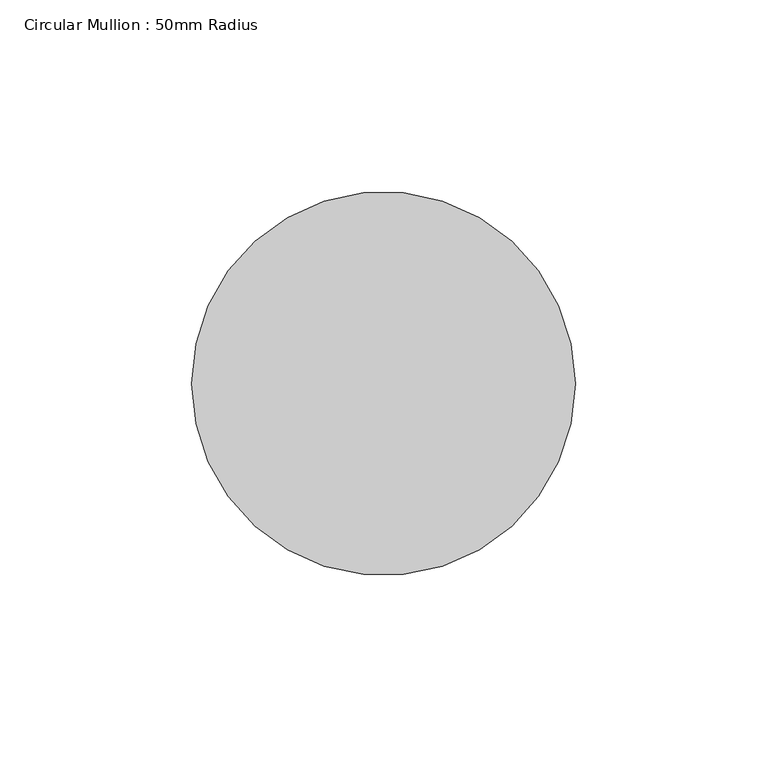
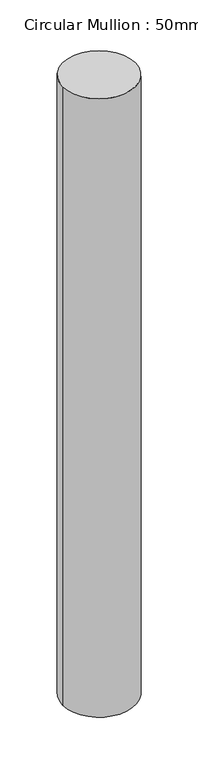
"""IFC4 building model written with IfcOpenShell, lengths in millimetres: member geometry, Circular Mullion : 50mm Radius."""

import ifcopenshell
import ifcopenshell.guid

model = None  # the IFC model being written
_history = None  # IfcOwnerHistory: only IFC2X3 demands one
_inside = {}  # id of a spatial element -> (the spatial element, [elements in it])
_under = {}  # id of a project, library or spatial element -> (it, [spatial elements below it])
_declared = {}  # id of a project -> (the project, [libraries it declares])
_typed = {}  # id of a type object -> (the type object, [elements of that type])
_made_of = {}  # id of a material, layer set ... -> (it, [elements and type objects made of it])


def new_model(schema):
    """Start an empty IFC model of exactly this schema.

    Asked for "IFC4X3", IfcOpenShell would pick the latest addendum, in which some entities
    have other attributes; the version numbers below select the first issue.
    IFC2X3 requires an IfcOwnerHistory on every rooted entity: one is made here for all.
    """
    global model, _history
    if schema == "IFC4X3":
        model = ifcopenshell.file(schema_version=(4, 3, 0, 0))
    else:
        model = ifcopenshell.file(schema=schema)
    _inside.clear()
    _under.clear()
    _declared.clear()
    _typed.clear()
    _made_of.clear()
    _history = None
    if model.schema == "IFC2X3":
        org = make("IfcOrganization", Name="unknown")
        user = make(
            "IfcPersonAndOrganization",
            ThePerson=make("IfcPerson", FamilyName="unknown"),
            TheOrganization=org,
        )
        app = make(
            "IfcApplication",
            ApplicationDeveloper=org,
            Version="unknown",
            ApplicationFullName="unknown",
            ApplicationIdentifier="unknown",
        )
        _history = make(
            "IfcOwnerHistory",
            OwningUser=user,
            OwningApplication=app,
            ChangeAction="ADDED",
            CreationDate=0,
        )
    return model


def make(cls, **values):
    """One entity of the class cls with the attributes given. An attribute that is None is left unset."""
    return model.create_entity(
        cls, **{name: value for name, value in values.items() if value is not None}
    )


def rooted(cls, **values):
    """An entity with a GlobalId (a new one), such as an element, a storey or a relation."""
    return make(cls, GlobalId=ifcopenshell.guid.new(), OwnerHistory=_history, **values)


def si_unit(unit_type, name, prefix=None):
    """IfcSIUnit, for example si_unit("LENGTHUNIT", "METRE", prefix="MILLI")."""
    return make("IfcSIUnit", UnitType=unit_type, Prefix=prefix, Name=name)


def assignment(units):
    """IfcUnitAssignment: the units of a project."""
    return None if units is None else make("IfcUnitAssignment", Units=units)


def point(xyz):
    """IfcCartesianPoint."""
    return None if xyz is None else make("IfcCartesianPoint", Coordinates=xyz)


def direction(xyz):
    """IfcDirection."""
    return None if xyz is None else make("IfcDirection", DirectionRatios=xyz)


def frame(location, z_axis=None, x_axis=None):
    """IfcAxis2Placement3D, a coordinate frame: its origin and axes. An axis left out is left unset."""
    return make(
        "IfcAxis2Placement3D",
        Location=point(location),
        Axis=direction(z_axis),
        RefDirection=direction(x_axis),
    )


def frame_2d(location, x_axis=None):
    """IfcAxis2Placement2D, a coordinate frame in the plane: its origin and x axis."""
    return make(
        "IfcAxis2Placement2D", Location=point(location), RefDirection=direction(x_axis)
    )


def origin():
    """The frame at (0, 0, 0) with its axes left unset."""
    return frame((0.0, 0.0, 0.0))


def origin_2d():
    """The frame at (0, 0) in the plane with its x axis left unset."""
    return frame_2d((0.0, 0.0))


def place(relative_to, where):
    """IfcLocalPlacement: puts the frame where relative to a parent placement (None: the world)."""
    return make(
        "IfcLocalPlacement", PlacementRelTo=relative_to, RelativePlacement=where
    )


def context(
    kind, dimensions, precision=None, world=None, true_north=None, identifier=None
):
    """IfcGeometricRepresentationContext, for example the 3D "Model" context."""
    return make(
        "IfcGeometricRepresentationContext",
        ContextIdentifier=identifier,
        ContextType=kind,
        CoordinateSpaceDimension=dimensions,
        Precision=precision,
        WorldCoordinateSystem=world,
        TrueNorth=true_north,
    )


def project(units=None, contexts=None):
    """IfcProject with its units and contexts."""
    return rooted(
        "IfcProject",
        Name="project",
        RepresentationContexts=contexts,
        UnitsInContext=assignment(units),
    )


def spatial(cls, under=None, at=None, **own):
    """A site, building, storey or space (cls), placed at a placement, below another one or the project."""
    s = rooted(cls, ObjectPlacement=at, **own)
    if under is not None:
        _under.setdefault(under.id(), (under, []))[1].append(s)
    return s


def circle_curve(where, radius):
    """IfcCircle in the frame where."""
    return make("IfcCircle", Position=where, Radius=radius)


def trimmed(basis, trim1, trim2, sense, master):
    """IfcTrimmedCurve: the piece of a basis curve between two trims."""
    return make(
        "IfcTrimmedCurve",
        BasisCurve=basis,
        Trim1=trim1,
        Trim2=trim2,
        SenseAgreement=sense,
        MasterRepresentation=master,
    )


def segment(curve, same_sense, transition):
    """IfcCompositeCurveSegment."""
    return make(
        "IfcCompositeCurveSegment",
        Transition=transition,
        SameSense=same_sense,
        ParentCurve=curve,
    )


def composite_curve(segments, self_intersect=None):
    """IfcCompositeCurve: segments joined end to end."""
    return make("IfcCompositeCurve", Segments=segments, SelfIntersect=self_intersect)


def outline(outer, holes=None, kind="AREA"):
    """IfcArbitraryClosedProfileDef: a profile drawn as a closed curve; with holes, ...WithVoids."""
    if holes is None:
        return make("IfcArbitraryClosedProfileDef", ProfileType=kind, OuterCurve=outer)
    return make(
        "IfcArbitraryProfileDefWithVoids",
        ProfileType=kind,
        OuterCurve=outer,
        InnerCurves=holes,
    )


def extrude(swept, where, along, depth):
    """IfcExtrudedAreaSolid: the profile swept, set in the frame where, extruded along a direction by depth."""
    return make(
        "IfcExtrudedAreaSolid",
        SweptArea=swept,
        Position=where,
        ExtrudedDirection=direction(along),
        Depth=depth,
    )


def shape(context_of_items, identifier, shape_type, items):
    """IfcShapeRepresentation: the items that make up one representation, for example the "Body"."""
    return make(
        "IfcShapeRepresentation",
        ContextOfItems=context_of_items,
        RepresentationIdentifier=identifier,
        RepresentationType=shape_type,
        Items=items,
    )


def source(mapping_origin, context_of_items, identifier, shape_type, items):
    """IfcRepresentationMap: a shape defined once, which mapped items show again and again."""
    return make(
        "IfcRepresentationMap",
        MappingOrigin=mapping_origin,
        MappedRepresentation=shape(context_of_items, identifier, shape_type, items),
    )


def transform(
    local_origin,
    x_axis=None,
    y_axis=None,
    z_axis=None,
    scale=None,
    scale2=None,
    scale3=None,
    uniform=True,
):
    """IfcCartesianTransformationOperator3D, or its non-uniform kind. x_axis, y_axis, z_axis: its Axis1, 2, 3."""
    if uniform:
        return make(
            "IfcCartesianTransformationOperator3D",
            Axis1=direction(x_axis),
            Axis2=direction(y_axis),
            LocalOrigin=point(local_origin),
            Scale=scale,
            Axis3=direction(z_axis),
        )
    return make(
        "IfcCartesianTransformationOperator3DnonUniform",
        Axis1=direction(x_axis),
        Axis2=direction(y_axis),
        LocalOrigin=point(local_origin),
        Scale=scale,
        Axis3=direction(z_axis),
        Scale2=scale2,
        Scale3=scale3,
    )


def mapped(mapping_source, mapping_target):
    """IfcMappedItem: shows the shape of a source again, moved by a transform."""
    return make(
        "IfcMappedItem", MappingSource=mapping_source, MappingTarget=mapping_target
    )


def made_of(thing, what):
    """Note that an element or type object is made of a material, layer set ...; save() writes the relation."""
    if what is not None:
        _made_of.setdefault(what.id(), (what, []))[1].append(thing)
    return thing


def element(
    cls,
    number,
    at=None,
    inside=None,
    cuts=None,
    type_object=None,
    material=None,
    context=None,
    identifier="Body",
    shape_type=None,
    held_by="IfcProductDefinitionShape",
    body=None,
    shapes=None,
    **own,
):
    """One element of the class cls, such as IfcWall. Its Tag is "e" and its number.

    at: its placement. inside: the storey or other place that contains it. cuts: it is an
    opening in that element (IfcRelVoidsElement). A single representation is given by context,
    identifier, shape_type and body (its items); several are given by shapes. held_by: the class
    of the entity that holds the representations. save() writes the other relations.
    """
    e = rooted(cls, Tag="e%d" % number, ObjectPlacement=at, **own)
    if body is not None:
        shapes = [shape(context, identifier, shape_type, body)]
    if shapes is not None:
        e.Representation = make(held_by, Representations=shapes)
    if inside is not None:
        _inside.setdefault(inside.id(), (inside, []))[1].append(e)
    if cuts is not None:
        rooted(
            "IfcRelVoidsElement", RelatingBuildingElement=cuts, RelatedOpeningElement=e
        )
    if type_object is not None:
        _typed.setdefault(type_object.id(), (type_object, []))[1].append(e)
    return made_of(e, material)


def aggregate(whole, parts):
    """IfcRelAggregates: a whole, such as a stair, and the parts it consists of."""
    return rooted("IfcRelAggregates", RelatingObject=whole, RelatedObjects=parts)


def save(model, path):
    """Write the relations noted so far, then the file.

    IfcRelAggregates (storeys below a building ...), IfcRelContainedInSpatialStructure (elements
    in a storey), IfcRelDefinesByType, IfcRelAssociatesMaterial and IfcRelDeclares: one each for
    every whole, place, type object, material and project.
    """
    for whole, parts in _under.values():
        aggregate(whole, parts)
    for where, things in _inside.values():
        rooted(
            "IfcRelContainedInSpatialStructure",
            RelatedElements=things,
            RelatingStructure=where,
        )
    for kind, things in _typed.values():
        rooted("IfcRelDefinesByType", RelatedObjects=things, RelatingType=kind)
    for what, things in _made_of.values():
        rooted("IfcRelAssociatesMaterial", RelatedObjects=things, RelatingMaterial=what)
    for by, libraries in _declared.values():
        rooted("IfcRelDeclares", RelatingContext=by, RelatedDefinitions=libraries)
    model.write(path)


def circular_mullion_50mm_radius_9237c12b(model_context):
    return source(origin(), model_context, "Body", "SweptSolid", [
        extrude(outline(composite_curve([segment(trimmed(circle_curve(origin_2d(), 50.0), [point((50.0, 0.0))], [point((-50.0, 0.0))], False, "CARTESIAN"), True, "CONTINUOUS"), segment(trimmed(circle_curve(origin_2d(), 50.0), [point((-50.0, 0.0))], [point((50.0, 0.0))], False, "CARTESIAN"), True, "CONTINUOUS")], self_intersect=False)), frame((0.0, 0.0, -900.1945123), z_axis=(0.0, 0.0, 1.0), x_axis=(1.0, 0.0, 0.0)), (0.0, 0.0, 1.0), 900.1945123),
    ])


if __name__ == "__main__":
    model = new_model("IFC4")
    model_context = context("Model", 3, world=origin())
    ifc_project = project(units=[si_unit("LENGTHUNIT", "METRE", prefix="MILLI")], contexts=[model_context])
    site = spatial("IfcSite", under=ifc_project)
    building = spatial("IfcBuilding", under=site)
    placement = place(None, origin())
    circular_mullion_50mm_radius_shape = circular_mullion_50mm_radius_9237c12b(model_context)
    element("IfcMember", 1, ObjectType="Circular Mullion : 50mm Radius", at=placement, inside=building, context=model_context, shape_type="MappedRepresentation", body=[
        mapped(circular_mullion_50mm_radius_shape, transform((0.0, 0.0, 0.0), x_axis=(1.0, 0.0, 0.0), y_axis=(0.0, 1.0, 0.0), z_axis=(0.0, 0.0, 1.0))),
    ])
    save(model, "model.ifc")

# Revit data of these elements
# Type "Circular Mullion : 50mm Radius"
#   built-in parameter 1007350 = 0.164042 (stored number, unit not read)
# Element 1 (IfcMember, "Circular Mullion : 50mm Radius")
#   Materials on its faces: "Aluminium"
# Materials
#   "Aluminium": class "Metal", colour RGB 247 247 247, transparency 0, Description = "Aluminium 6061", Cost = 0
